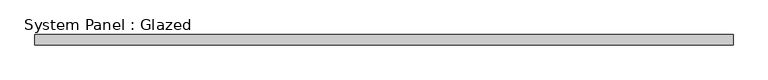
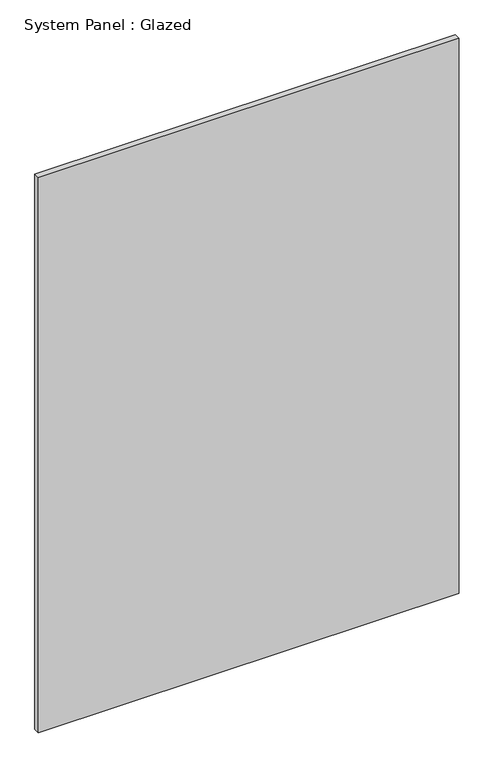
"""IFC4 building model written with IfcOpenShell, lengths in millimetres: plate geometry, System Panel : Glazed."""

from ifc_helpers import new_model, si_unit, origin, origin_with_axes, place, context, project, spatial, polyline, outline, extrude, source, transform, mapped, element, save


def system_panel_glazed_c7b2fa33(model_context):
    return source(origin(), model_context, "Body", "SweptSolid", [
        extrude(outline(polyline([(851.3636364, 24.5), (-851.3636364, 24.5), (-851.3636364, 49.5), (851.3636364, 49.5), (851.3636364, 24.5)])), origin_with_axes(), (0.0, 0.0, 1.0), 2375.0),
    ])


if __name__ == "__main__":
    model = new_model("IFC4")
    model_context = context("Model", 3, world=origin())
    ifc_project = project(units=[si_unit("LENGTHUNIT", "METRE", prefix="MILLI")], contexts=[model_context])
    site = spatial("IfcSite", under=ifc_project)
    building = spatial("IfcBuilding", under=site)
    placement = place(None, origin())
    system_panel_glazed_shape = system_panel_glazed_c7b2fa33(model_context)
    element("IfcPlate", 1, ObjectType="System Panel : Glazed", at=placement, inside=building, context=model_context, shape_type="MappedRepresentation", body=[
        mapped(system_panel_glazed_shape, transform((0.0, 0.0, 0.0), x_axis=(1.0, 0.0, 0.0), y_axis=(0.0, 1.0, 0.0), z_axis=(0.0, 0.0, 1.0))),
    ])
    save(model, "model.ifc")

# Revit data of these elements
# Element 1 (IfcPlate, "System Panel : Glazed")
#   Materials on its faces: "Glass"
# Materials
#   "Glass": class "Glass", colour RGB 218 227 224, transparency 0.85, Description = "Soda Lime Glass", Cost = 0
